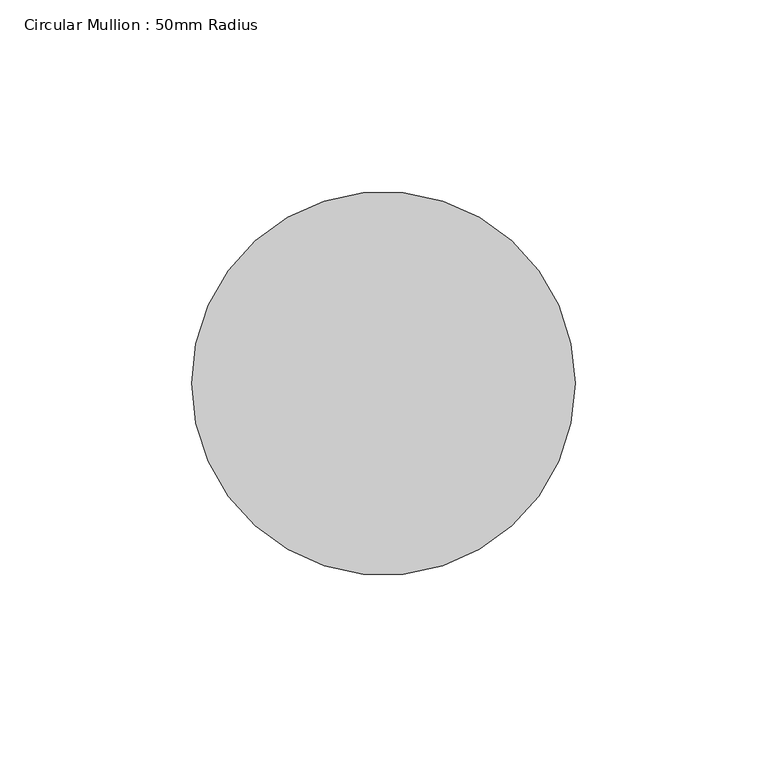
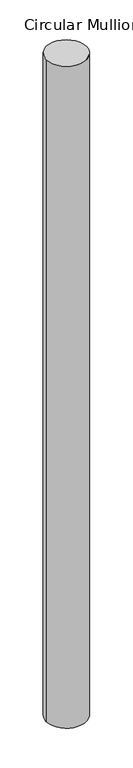
"""IFC4 building model written with IfcOpenShell, lengths in millimetres: member geometry, Circular Mullion : 50mm Radius."""

from ifc_helpers import new_model, si_unit, point, frame, origin, origin_2d, place, context, project, spatial, circle_curve, trimmed, segment, composite_curve, outline, extrude, source, transform, mapped, element, save


def circular_mullion_50mm_radius_e23fd9d7(model_context):
    return source(origin(), model_context, "Body", "SweptSolid", [
        extrude(outline(composite_curve([segment(trimmed(circle_curve(origin_2d(), 50.0), [point((50.0, 0.0))], [point((-50.0, 0.0))], False, "CARTESIAN"), True, "CONTINUOUS"), segment(trimmed(circle_curve(origin_2d(), 50.0), [point((-50.0, 0.0))], [point((50.0, 0.0))], False, "CARTESIAN"), True, "CONTINUOUS")], self_intersect=False)), frame((0.0, 0.0, -1746.2816529), z_axis=(0.0, 0.0, 1.0), x_axis=(1.0, 0.0, 0.0)), (0.0, 0.0, 1.0), 1746.2816529),
    ])


if __name__ == "__main__":
    model = new_model("IFC4")
    model_context = context("Model", 3, world=origin())
    ifc_project = project(units=[si_unit("LENGTHUNIT", "METRE", prefix="MILLI")], contexts=[model_context])
    site = spatial("IfcSite", under=ifc_project)
    building = spatial("IfcBuilding", under=site)
    placement = place(None, origin())
    circular_mullion_50mm_radius_shape = circular_mullion_50mm_radius_e23fd9d7(model_context)
    element("IfcMember", 1, ObjectType="Circular Mullion : 50mm Radius", at=placement, inside=building, context=model_context, shape_type="MappedRepresentation", body=[
        mapped(circular_mullion_50mm_radius_shape, transform((0.0, 0.0, 0.0), x_axis=(1.0, 0.0, 0.0), y_axis=(0.0, 1.0, 0.0), z_axis=(0.0, 0.0, 1.0))),
    ])
    save(model, "model.ifc")

# Revit data of these elements
# Type "Circular Mullion : 50mm Radius"
#   built-in parameter 1007350 = 0.164042 (stored number, unit not read)
# Element 1 (IfcMember, "Circular Mullion : 50mm Radius")
#   Materials on its faces: "Aluminium"
# Materials
#   "Aluminium": class "Metal", colour RGB 247 247 247, transparency 0, Description = "Aluminium 6061", Cost = 0
